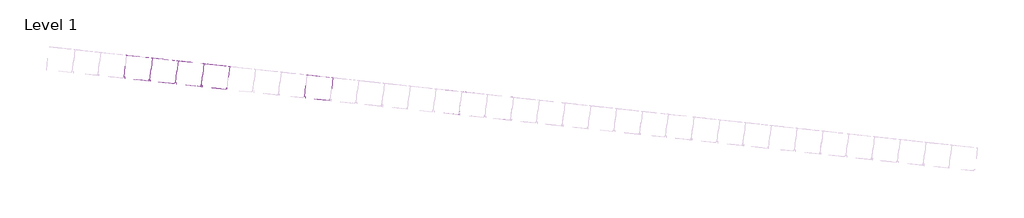
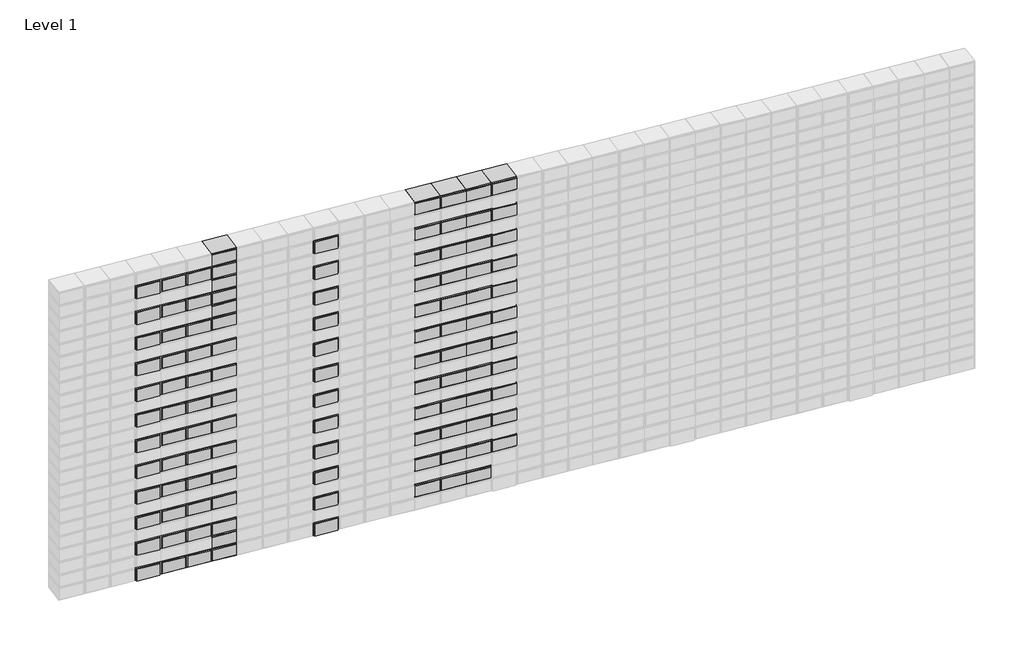
# One storey, part 13 of 18: 111 proxies.
# Revit data of these elements (continued)
# Elements 29, 30, 31, 32, 33, 34, 35, 36, 37, 38, 39, 40, 41, 42, 43, 44, 45, 46, 47, 48, 49, 50, 51 (IfcBuildingElementProxy, "00_GMA_steen_versie_6 : Geel") (continued)
#   LintVoegBovenHalf = 5 mm
#   LintVoegBoven = 10 mm
#   Phase Created = New Construction
#   Materials on its faces: "20_voeg", "21_steen_geel"
# Elements 52, 53, 54, 55, 56, 57, 58, 59, 60, 61, 62, 63, 64, 65, 66, 67, 68, 69, 70, 71, 72, 73, 74, 75, 76, 77, 78, 79, 80, 81, 82, 83, 84, 85, 86, 87 (IfcBuildingElementProxy, "00_GMA_steen_versie_6 : Rood")
#   StootvoegLinksHalfOnder = 5 mm
#   StootvoegLinksHalfBoven = 5 mm
#   StootVoegRechtsHalfOnder = 5 mm
#   StootVoegRechtsHalfBoven = 5 mm
#   StootVoegBreedteRechts = 10 mm
#   StootVoegBreedteLinks = 10 mm
#   LintVoegOnderHalf = 5 mm
#   LintVoegOnder = 10 mm
#   LintVoegBovenHalf = 5 mm
#   LintVoegBoven = 10 mm
#   Phase Created = New Construction
#   Materials on its faces: "20_voeg", "21_steen_rood"
# Elements 88, 89, 90, 91, 92, 93, 94, 95, 96, 97, 98, 99, 100, 101, 102, 103, 104, 105, 106, 107, 108, 109, 110, 111 (IfcBuildingElementProxy, "00_GMA_steen_versie_6 : Rood")
#   StootvoegLinksHalfOnder = 5 mm
#   StootvoegLinksHalfBoven = 5 mm
#   StootVoegRechtsHalfOnder = 5 mm
#   StootVoegRechtsHalfBoven = 5 mm
#   StootVoegBreedteRechts = 10 mm
#   StootVoegBreedteLinks = 10 mm
#   LintVoegOnderHalf = 0 mm
#   LintVoegOnder = 0 mm
#   LintVoegBovenHalf = 5 mm
#   LintVoegBoven = 10 mm
#   Phase Created = New Construction
#   Materials on its faces: "20_voeg", "21_steen_rood"
# Materials
#   "21_steen_geel": class "Unassigned", colour RGB 202 202 0, transparency 0, Cost = 0
#   "20_voeg": class "Concrete", colour RGB 86 86 86, transparency 0, Manufacturer = "RevitGG", URL = "www.revitgg.nl", Description = "zandcement, generiek materiaal", Cost = 0
#   "21_steen_rood": class "Unassigned", colour RGB 213 111 43, transparency 0, Cost = 0
